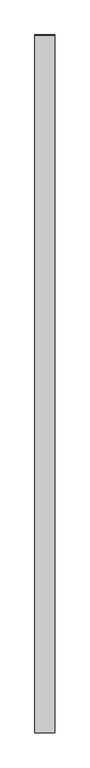
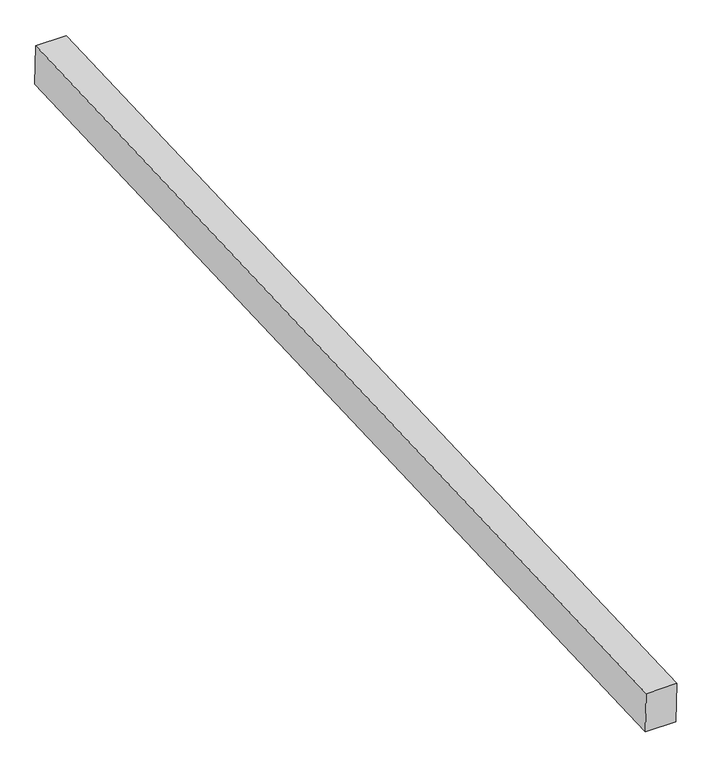
"""IFC4 building model written with IfcOpenShell, lengths in millimetres: proxy geometry, Generic Models 7:Generic Models 1:8:Generic Models 1:8 : Generic Models 7:Generic Models 1:337419:13 : Generic Models 7:Generic Models 1:8:Generic Models 1:8 : Generic Models 7:Generic Models 1:337419:315935."""

from ifc_helpers import new_model, si_unit, frame, origin, place, context, project, spatial, polyline, outline, extrude, source, transform, mapped, element, save


def generic_models_481e84af(model_context):
    return source(origin(), model_context, "Body", "SweptSolid", [
        extrude(outline(polyline([(-580626.5557381, 3844.0209448), (-575753.6328438, 4047.0593987), (-575746.0659221, 3856.7093942), (-580618.6251193, 3653.6860944), (-580626.5557381, 3844.0209448)])), frame((596116.161724, 0.0, 0.0), z_axis=(1.0, 0.0, 0.0), x_axis=(0.0, 1.0, 0.0)), (0.0, 0.0, 1.0), 139.7),
    ])


if __name__ == "__main__":
    model = new_model("IFC4")
    model_context = context("Model", 3, world=origin())
    ifc_project = project(units=[si_unit("LENGTHUNIT", "METRE", prefix="MILLI")], contexts=[model_context])
    site = spatial("IfcSite", under=ifc_project)
    building = spatial("IfcBuilding", under=site)
    placement = place(None, origin())
    generic_models_shape = generic_models_481e84af(model_context)
    element("IfcBuildingElementProxy", 1, Name="Generic Models 7:Generic Models 1:8:Generic Models 1:8 : Generic Models 7:Generic Models 1:337419:13 : Generic Models 7:Generic Models 1:8:Generic Models 1:8 : Generic Models 7:Generic Models 1:337419:315935", ObjectType="Generic Models 7:Generic Models 1:8:Generic Models 1:8 : Generic Models 7:Generic Models 1:337419:13 : Generic Models 7:Generic Models 1:8:Generic Models 1:8 : Generic Models 7:Generic Models 1:337419:315935", at=placement, inside=building, context=model_context, shape_type="MappedRepresentation", body=[
        mapped(generic_models_shape, transform((0.0, 0.0, 0.0), x_axis=(1.0, 0.0, 0.0), y_axis=(0.0, 1.0, 0.0), z_axis=(0.0, 0.0, 1.0))),
    ])
    save(model, "model.ifc")

# Revit data of these elements
# Type "Generic Models 7:Generic Models 1:8:Generic Models 1:8 : Generic Models 7:Generic Models 1:337419:13 : Generic Models 7:Generic Models 1:8:Generic Models 1:8 : Generic Models 7:Generic Models 1:337419:315935"
#   NameOverride = "Generic Models 7:Generic Models 1:8:Generic Models 1:8 : Generic Models 7:Generic Models 1:337419:315935"
#   ObjectTypeOverride = "Generic Models 1:8 : Generic Models 7:Generic Models 1:337419"
#   Reference = "Generic Models 1"
#   Tag = "315935"
# Element 1 (IfcBuildingElementProxy, "Generic Models 7:Generic Models 1:8:Generic Models 1:8 : Generic Models 7:Generic Models 1:337419:13 : Generic Models 7:Generic Models 1:8:Generic Models 1:8 : Generic Models 7:Generic Models 1:337419:315935")
#   Materials on its faces: "5 1/2\" X 7 1/2\" EXTERIOR GRADE GLULAM BEAMS"
# Materials
#   "5 1/2\" X 7 1/2\" EXTERIOR GRADE GLULAM BEAMS": class "Wood", colour RGB 183 134 68, transparency 0, Keynote = "M06181300.01", Description = "Pinus Echinata", Cost = 0
